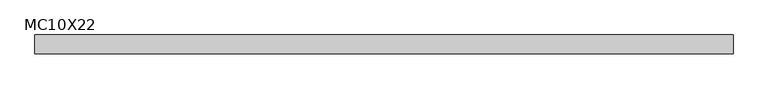
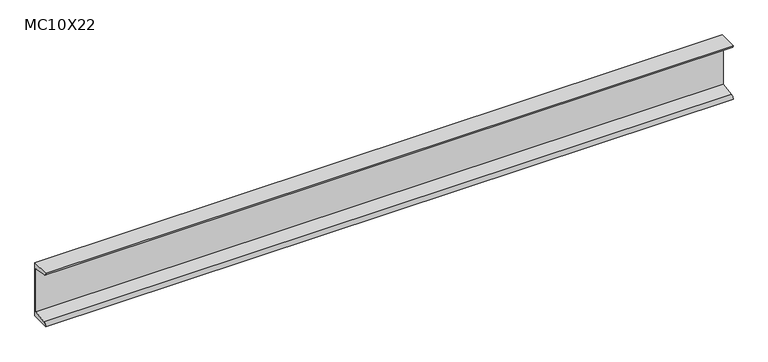
"""IFC4 building model written with IfcOpenShell, lengths in millimetres: beam geometry, MC-Miscellaneous Channel : MC10X22."""

from ifc_helpers import new_model, si_unit, point, frame, frame_2d, origin, place, context, project, spatial, polyline, circle_curve, trimmed, segment, composite_curve, outline, extrude, source, transform, mapped, element, save


def mc10x22_b79fa394(model_context):
    return source(origin(), model_context, "Body", "SweptSolid", [
        extrude(outline(composite_curve([segment(polyline([(25.146, 127.0), (25.146, -127.0), (-59.182, -127.0)]), True, "CONTINUOUS"), segment(trimmed(circle_curve(frame_2d((-44.577, -127.0)), 14.605), [point((-59.182, -127.0))], [point((-44.577, -112.395))], False, "CARTESIAN"), True, "CONTINUOUS"), segment(polyline([(-44.577, -112.395), (17.78, -102.5186215), (17.78, 102.5186215), (-44.577, 112.395)]), True, "CONTINUOUS"), segment(trimmed(circle_curve(frame_2d((-44.577, 127.0)), 14.605), [point((-44.577, 112.395))], [point((-59.182, 127.0))], False, "CARTESIAN"), True, "CONTINUOUS"), segment(polyline([(-59.182, 127.0), (25.146, 127.0)]), True, "CONTINUOUS")], self_intersect=False)), frame((-1547.5239638, 0.0, 0.0), z_axis=(1.0, 0.0, 0.0), x_axis=(0.0, 1.0, 0.0)), (0.0, 0.0, 1.0), 3095.0479276),
    ])


if __name__ == "__main__":
    model = new_model("IFC4")
    model_context = context("Model", 3, world=origin())
    ifc_project = project(units=[si_unit("LENGTHUNIT", "METRE", prefix="MILLI")], contexts=[model_context])
    site = spatial("IfcSite", under=ifc_project)
    building = spatial("IfcBuilding", under=site)
    placement = place(None, origin())
    mc10x22_shape = mc10x22_b79fa394(model_context)
    element("IfcBeam", 1, ObjectType="MC-Miscellaneous Channel : MC10X22", at=placement, inside=building, context=model_context, shape_type="MappedRepresentation", body=[
        mapped(mc10x22_shape, transform((0.0, 0.0, 0.0), x_axis=(1.0, 0.0, 0.0), y_axis=(0.0, 1.0, 0.0), z_axis=(0.0, 0.0, 1.0))),
    ])
    save(model, "model.ifc")

# Revit data of these elements
# Type "MC-Miscellaneous Channel : MC10X22"
#   Assembly Code = "B10"
#   W = 22
#   Length [instance default] = 5' - 0"
#   bf = 0' - 3.32"
#   d = 0' - 10"
#   tf = 0' - 0.575"
#   tw = 0' - 0.29"
#   x = 0' - 0.99"
#   A = 0.0447917 SF
#   Structural Material [instance default] = Steel ASTM A36
# Element 1 (IfcBeam, "MC-Miscellaneous Channel : MC10X22")
#   Length = 10' - 1.85228"
#   Structural Material = Metal - Steel - ASTM A992
#   Materials on its faces: "Metal - Steel - ASTM A992"
# Materials
#   "Steel ASTM A36": class "Metal", colour RGB 199 199 199, transparency 0, Description = "Structural steel, ASTM A36 Grade B, mill finish", Cost = 0
#   "Metal - Steel - ASTM A992": class "Metal", colour RGB 255 128 0, transparency 0
